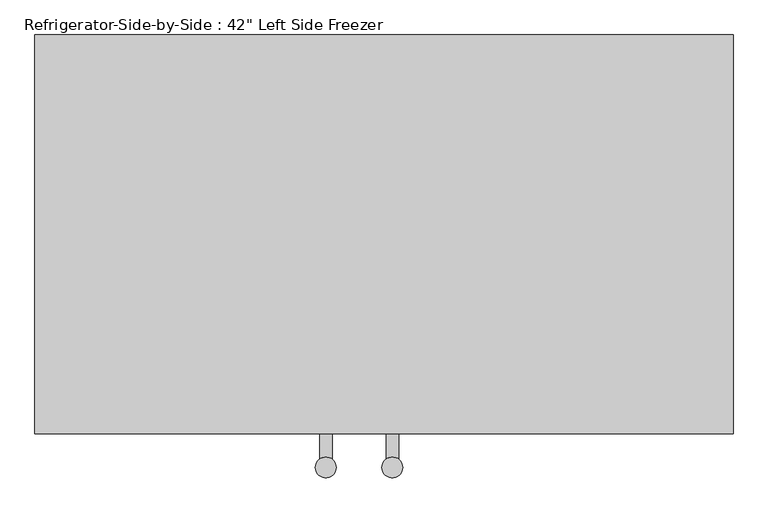
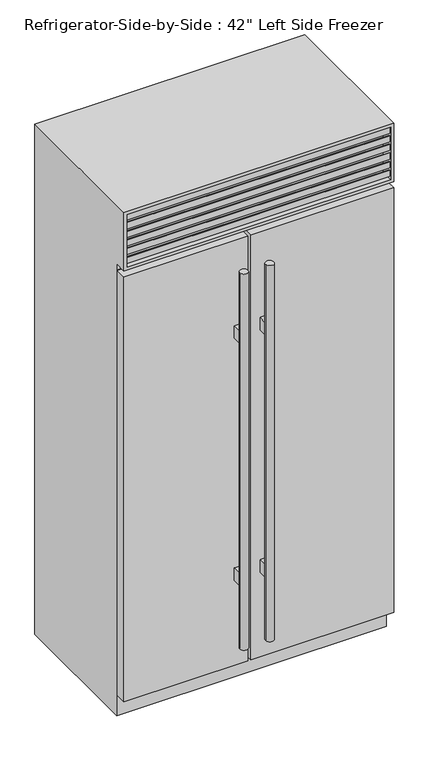
"""IFC4 building model written with IfcOpenShell, lengths in millimetres: proxy geometry."""

from ifc_helpers import new_model, si_unit, frame, origin, place, context, project, spatial, polyline, circle_curve, ellipse_curve, outline, extrude, faceted_brep, source, transform, mapped, element, save
from ifc_brep_helpers import plane_surface, cylinder_surface, advanced_brep


def proxy_0447ab4b(model_context):
    return source(origin(), model_context, "Body", "SolidModel", [
        extrude(outline(polyline([(-533.4, -666.75), (-44.45, -666.75), (-44.45, -711.2), (-533.4, -711.2), (-533.4, -666.75)])), frame((0.0, 0.0, 88.9), z_axis=(0.0, 0.0, 1.0), x_axis=(1.0, 0.0, 0.0)), (0.0, 0.0, 1.0), 1774.825),
        extrude(outline(polyline([(-31.75, -666.75), (533.4, -666.75), (533.4, -711.2), (-31.75, -711.2), (-31.75, -666.75)])), frame((0.0, 0.0, 88.9), z_axis=(0.0, 0.0, 1.0), x_axis=(1.0, 0.0, 0.0)), (0.0, 0.0, 1.0), 1774.825),
        faceted_brep([(533.4, -711.2, 2133.6), (-533.4, -711.2, 2133.6), (-533.4, -711.2, 1889.125), (533.4, -711.2, 1889.125), (520.7, -711.2, 2120.9), (520.7, -711.2, 1901.825), (-520.7, -711.2, 1901.825), (-520.7, -711.2, 2120.9), (533.4, -101.6, 2133.6), (-533.4, -101.6, 2133.6), (-533.4, -101.6, 0.0), (-533.4, -660.4, 0.0), (-533.4, -660.4, 1889.125), (533.4, -660.4, 1889.125), (533.4, -660.4, 0.0), (533.4, -101.6, 0.0), (-520.7, -660.4, 2120.9), (520.7, -660.4, 2120.9), (-520.7, -660.4, 1901.825), (520.7, -660.4, 1901.825)], [[[0, 1, 2, 3], [4, 5, 6, 7]], [[1, 0, 8, 9]], [[2, 1, 9, 10, 11, 12]], [[3, 2, 12, 13]], [[8, 0, 3, 13, 14, 15]], [[4, 7, 16, 17]], [[7, 6, 18, 16]], [[6, 5, 19, 18]], [[5, 4, 17, 19]], [[15, 14, 11, 10]], [[9, 8, 15, 10]], [[17, 16, 18, 19]], [[11, 14, 13, 12]]]),
        extrude(outline(polyline([(-660.4, 1901.825), (-708.025, 1914.5860803), (-708.025, 1939.9860803), (-704.85, 1939.9860803), (-704.85, 1917.1368938), (-660.4, 1905.2265522), (-660.4, 1901.825)])), frame((-520.7, 0.0, 0.0), z_axis=(1.0, 0.0, 0.0), x_axis=(0.0, 1.0, 0.0)), (0.0, 0.0, 1.0), 1041.4),
        extrude(outline(polyline([(-660.4, 1938.0077839), (-708.025, 1950.7688642), (-708.025, 1976.1688642), (-704.85, 1976.1688642), (-704.85, 1953.3196777), (-660.4, 1941.4093361), (-660.4, 1938.0077839)])), frame((-520.7, 0.0, 0.0), z_axis=(1.0, 0.0, 0.0), x_axis=(0.0, 1.0, 0.0)), (0.0, 0.0, 1.0), 1041.4),
        extrude(outline(polyline([(-660.4, 1974.1905679), (-708.025, 1986.9516482), (-708.025, 2012.3516482), (-704.85, 2012.3516482), (-704.85, 1989.5024616), (-660.4, 1977.59212), (-660.4, 1974.1905679)])), frame((-520.7, 0.0, 0.0), z_axis=(1.0, 0.0, 0.0), x_axis=(0.0, 1.0, 0.0)), (0.0, 0.0, 1.0), 1041.4),
        extrude(outline(polyline([(-660.4, 2010.3733518), (-708.025, 2023.1344321), (-708.025, 2048.5344321), (-704.85, 2048.5344321), (-704.85, 2025.6852456), (-660.4, 2013.774904), (-660.4, 2010.3733518)])), frame((-520.7, 0.0, 0.0), z_axis=(1.0, 0.0, 0.0), x_axis=(0.0, 1.0, 0.0)), (0.0, 0.0, 1.0), 1041.4),
        extrude(outline(polyline([(-660.4, 2046.5561358), (-708.025, 2059.3172161), (-708.025, 2084.7172161), (-704.85, 2084.7172161), (-704.85, 2061.8680295), (-660.4, 2049.9576879), (-660.4, 2046.5561358)])), frame((-520.7, 0.0, 0.0), z_axis=(1.0, 0.0, 0.0), x_axis=(0.0, 1.0, 0.0)), (0.0, 0.0, 1.0), 1041.4),
        extrude(outline(polyline([(-660.4, 2082.7389197), (-708.025, 2095.5), (-708.025, 2120.9), (-704.85, 2120.9), (-704.85, 2098.0508135), (-660.4, 2086.1404719), (-660.4, 2082.7389197)])), frame((-520.7, 0.0, 0.0), z_axis=(1.0, 0.0, 0.0), x_axis=(0.0, 1.0, 0.0)), (0.0, 0.0, 1.0), 1041.4),
        advanced_brep(
        [(-25.4, -660.4, 1857.375), (-25.4, -666.75, 1857.375), (-25.4, -666.75, 95.25), (-25.4, -660.4, 95.25), (527.05, -666.75, 95.25), (527.05, -660.4, 95.25), (527.05, -666.75, 1857.375), (527.05, -660.4, 1857.375), (-28.575, -660.4, 1860.55), (530.225, -660.4, 1860.55), (530.225, -660.4, 92.075), (-28.575, -660.4, 92.075), (-28.575, -666.75, 92.075), (530.225, -666.75, 92.075), (530.225, -666.75, 1860.55), (-28.575, -666.75, 1860.55)],
        [
            (0, 1),
            (1, 2),
            (2, 3),
            (3, 0),
            (2, 4),
            (4, 5),
            (5, 3),
            (4, 6),
            (6, 7),
            (7, 5),
            (8, 9),
            (9, 10),
            (10, 11),
            (11, 8),
            (7, 0),
            (12, 13),
            (13, 14),
            (14, 15),
            (15, 12),
            (1, 6),
            (15, 8, ellipse_curve(frame((-28.575, -663.575, 1860.55), z_axis=(-0.7071067811865415, 0.0, -0.7071067811865537), x_axis=(-0.7071067811865536, 0.0, 0.7071067811865414)), 4.4901281, 3.175)),
            (11, 12, ellipse_curve(frame((-28.575, -663.575, 92.075), z_axis=(-0.7071067811865598, 0.0, 0.7071067811865352), x_axis=(0.7071067811865352, 0.0, 0.7071067811865598)), 4.4901281, 3.175)),
            (10, 13, ellipse_curve(frame((530.225, -663.575, 92.075), z_axis=(-0.7071067811865352, 0.0, -0.7071067811865598), x_axis=(-0.7071067811865598, 0.0, 0.7071067811865352)), 4.4901281, 3.175)),
            (9, 14, ellipse_curve(frame((530.225, -663.575, 1860.55), z_axis=(0.7071067811865536, 0.0, -0.7071067811865412), x_axis=(-0.7071067811865411, 0.0, -0.7071067811865539)), 4.4901281, 3.175)),
        ],
        [
            plane_surface(frame((-25.4, -666.75, 1857.375), z_axis=(1.0, 0.0, 0.0), x_axis=(0.0, 0.0, -1.0))),
            plane_surface(frame((-25.4, -666.75, 95.25), z_axis=(0.0, 0.0, 1.0), x_axis=(1.0, 0.0, 0.0))),
            plane_surface(frame((527.05, -666.75, 95.25), z_axis=(-1.0, 0.0, 0.0), x_axis=(0.0, 0.0, 1.0))),
            plane_surface(frame((527.05, -660.4, 1857.375), z_axis=(0.0, 1.0, 0.0), x_axis=(-1.0, 0.0, 0.0))),
            plane_surface(frame((530.225, -666.75, 1860.55), z_axis=(0.0, -1.0, 0.0), x_axis=(-1.0, 0.0, 0.0))),
            plane_surface(frame((527.05, -666.75, 1857.375), z_axis=(0.0, 0.0, -1.0), x_axis=(-1.0, 0.0, 0.0))),
            cylinder_surface(frame((-28.575, -663.575, 1863.725), z_axis=(0.0, 0.0, 1.0), x_axis=(0.0, -1.0, 0.0)), 3.175),
            cylinder_surface(frame((-31.75, -663.575, 92.075), z_axis=(-1.0, 0.0, 0.0), x_axis=(0.0, -1.0, 0.0)), 3.175),
            cylinder_surface(frame((530.225, -663.575, 88.9), z_axis=(0.0, 0.0, -1.0), x_axis=(0.0, -1.0, 0.0)), 3.175),
            cylinder_surface(frame((533.4, -663.575, 1860.55), z_axis=(1.0, 0.0, 0.0), x_axis=(0.0, -1.0, 0.0)), 3.175),
        ],
        [
            (0, [[1, 2, 3, 4]]),
            (1, [[-3, 5, 6, 7]]),
            (2, [[-6, 8, 9, 10]]),
            (3, [[11, 12, 13, 14], [-7, -10, 15, -4]]),
            (4, [[16, 17, 18, 19], [20, -8, -5, -2]]),
            (5, [[-9, -20, -1, -15]]),
            (6, [[21, -14, 22, -19]]),
            (7, [[-22, -13, 23, -16]]),
            (8, [[-23, -12, 24, -17]]),
            (9, [[-24, -11, -21, -18]]),
        ],
    ),
        advanced_brep(
        [(-527.05, -660.4, 1857.375), (-527.05, -666.75, 1857.375), (-527.05, -666.75, 95.25), (-527.05, -660.4, 95.25), (-50.8, -666.75, 95.25), (-50.8, -660.4, 95.25), (-50.8, -666.75, 1857.375), (-50.8, -660.4, 1857.375), (-530.225, -660.4, 1860.55), (-47.625, -660.4, 1860.55), (-47.625, -660.4, 92.075), (-530.225, -660.4, 92.075), (-530.225, -666.75, 92.075), (-47.625, -666.75, 92.075), (-47.625, -666.75, 1860.55), (-530.225, -666.75, 1860.55)],
        [
            (0, 1),
            (1, 2),
            (2, 3),
            (3, 0),
            (2, 4),
            (4, 5),
            (5, 3),
            (4, 6),
            (6, 7),
            (7, 5),
            (8, 9),
            (9, 10),
            (10, 11),
            (11, 8),
            (7, 0),
            (12, 13),
            (13, 14),
            (14, 15),
            (15, 12),
            (1, 6),
            (15, 8, ellipse_curve(frame((-530.225, -663.575, 1860.55), z_axis=(-0.7071067811865475, 0.0, -0.7071067811865475), x_axis=(-0.7071067811865474, 0.0, 0.7071067811865476)), 4.4901281, 3.175)),
            (11, 12, ellipse_curve(frame((-530.225, -663.575, 92.075), z_axis=(-0.7071067811865475, 0.0, 0.7071067811865475), x_axis=(0.7071067811865474, 0.0, 0.7071067811865476)), 4.4901281, 3.175)),
            (10, 13, ellipse_curve(frame((-47.625, -663.575, 92.075), z_axis=(-0.7071067811865475, 0.0, -0.7071067811865475), x_axis=(-0.7071067811865476, 0.0, 0.7071067811865474)), 4.4901281, 3.175)),
            (9, 14, ellipse_curve(frame((-47.625, -663.575, 1860.55), z_axis=(0.7071067811865475, 0.0, -0.7071067811865475), x_axis=(-0.7071067811865474, 0.0, -0.7071067811865476)), 4.4901281, 3.175)),
        ],
        [
            plane_surface(frame((-527.05, -666.75, 1857.375), z_axis=(1.0, 0.0, 0.0), x_axis=(0.0, 0.0, -1.0))),
            plane_surface(frame((-527.05, -666.75, 95.25), z_axis=(0.0, 0.0, 1.0), x_axis=(1.0, 0.0, 0.0))),
            plane_surface(frame((-50.8, -666.75, 95.25), z_axis=(-1.0, 0.0, 0.0), x_axis=(0.0, 0.0, 1.0))),
            plane_surface(frame((-50.8, -660.4, 1857.375), z_axis=(0.0, 1.0, 0.0), x_axis=(-1.0, 0.0, 0.0))),
            plane_surface(frame((-47.625, -666.75, 1860.55), z_axis=(0.0, -1.0, 0.0), x_axis=(-1.0, 0.0, 0.0))),
            plane_surface(frame((-50.8, -666.75, 1857.375), z_axis=(0.0, 0.0, -1.0), x_axis=(-1.0, 0.0, 0.0))),
            cylinder_surface(frame((-530.225, -663.575, 1863.725), z_axis=(0.0, 0.0, 1.0), x_axis=(0.0, -1.0, 0.0)), 3.175),
            cylinder_surface(frame((-533.4, -663.575, 92.075), z_axis=(-1.0, 0.0, 0.0), x_axis=(0.0, -1.0, 0.0)), 3.175),
            cylinder_surface(frame((-47.625, -663.575, 88.9), z_axis=(0.0, 0.0, -1.0), x_axis=(0.0, -1.0, 0.0)), 3.175),
            cylinder_surface(frame((-44.45, -663.575, 1860.55), z_axis=(1.0, 0.0, 0.0), x_axis=(0.0, -1.0, 0.0)), 3.175),
        ],
        [
            (0, [[1, 2, 3, 4]]),
            (1, [[-3, 5, 6, 7]]),
            (2, [[-6, 8, 9, 10]]),
            (3, [[11, 12, 13, 14], [-7, -10, 15, -4]]),
            (4, [[16, 17, 18, 19], [20, -8, -5, -2]]),
            (5, [[-9, -20, -1, -15]]),
            (6, [[21, -14, 22, -19]]),
            (7, [[-22, -13, 23, -16]]),
            (8, [[-23, -12, 24, -17]]),
            (9, [[-24, -11, -21, -18]]),
        ],
    ),
        advanced_brep(
        [(-3.175, -762.3741958, 1762.125), (28.575, -762.3741958, 1762.125), (-3.175, -762.3741958, 190.5), (28.575, -762.3741958, 190.5), (22.225, -749.6741958, 1457.325), (22.225, -749.6741958, 1508.125), (3.175, -749.6741958, 1508.125), (3.175, -749.6741958, 1457.325), (22.225, -749.6741958, 444.5), (22.225, -749.6741958, 495.3), (3.175, -749.6741958, 495.3), (3.175, -749.6741958, 444.5), (22.225, -711.2, 1508.125), (22.225, -711.2, 1457.325), (3.175, -711.2, 1457.325), (3.175, -711.2, 1508.125), (22.225, -711.2, 495.3), (22.225, -711.2, 444.5), (3.175, -711.2, 444.5), (3.175, -711.2, 495.3)],
        [
            (0, 1, circle_curve(frame((12.7, -762.3741958, 1762.125), z_axis=(0.0, 0.0, 1.0), x_axis=(1.0, 0.0, 0.0)), 15.875)),
            (1, 0, circle_curve(frame((12.7, -762.3741958, 1762.125), z_axis=(0.0, 0.0, 1.0), x_axis=(1.0, 0.0, 0.0)), 15.875)),
            (2, 3, circle_curve(frame((12.7, -762.3741958, 190.5), z_axis=(0.0, 0.0, -1.0), x_axis=(1.0, 0.0, 0.0)), 15.875)),
            (3, 2, circle_curve(frame((12.7, -762.3741958, 190.5), z_axis=(0.0, 0.0, -1.0), x_axis=(1.0, 0.0, 0.0)), 15.875)),
            (0, 2),
            (3, 1),
            (4, 5),
            (5, 6, circle_curve(frame((12.7, -762.3741958, 1508.125), z_axis=(0.0, 0.0, 1.0), x_axis=(1.0, 0.0, 0.0)), 15.875)),
            (6, 7),
            (7, 4, circle_curve(frame((12.7, -762.3741958, 1457.325), z_axis=(0.0, 0.0, -1.0), x_axis=(1.0, 0.0, 0.0)), 15.875)),
            (8, 9),
            (9, 10, circle_curve(frame((12.7, -762.3741958, 495.3), z_axis=(0.0, 0.0, 1.0), x_axis=(1.0, 0.0, 0.0)), 15.875)),
            (10, 11),
            (11, 8, circle_curve(frame((12.7, -762.3741958, 444.5), z_axis=(0.0, 0.0, -1.0), x_axis=(1.0, 0.0, 0.0)), 15.875)),
            (12, 13),
            (13, 14),
            (14, 15),
            (15, 12),
            (16, 17),
            (17, 18),
            (18, 19),
            (19, 16),
            (12, 5),
            (4, 13),
            (7, 14),
            (6, 15),
            (16, 9),
            (8, 17),
            (11, 18),
            (10, 19),
        ],
        [
            plane_surface(frame((28.575, -762.3741958, 1762.125), z_axis=(0.0, 0.0, 1.0), x_axis=(0.0, 1.0, 0.0))),
            plane_surface(frame((28.575, -762.3741958, 190.5), z_axis=(0.0, 0.0, -1.0), x_axis=(0.0, -1.0, 0.0))),
            cylinder_surface(frame((12.7, -762.3741958, 190.5), z_axis=(0.0, 0.0, 1.0), x_axis=(1.0, 0.0, 0.0)), 15.875),
            plane_surface(frame((22.225, -711.2, 1508.125), z_axis=(0.0, 1.0, 0.0), x_axis=(0.0, 0.0, -1.0))),
            plane_surface(frame((22.225, -711.2, 1508.125), z_axis=(1.0, 0.0, 0.0), x_axis=(0.0, -1.0, 0.0))),
            plane_surface(frame((22.225, -711.2, 1457.325), z_axis=(0.0, 0.0, -1.0), x_axis=(0.0, -1.0, 0.0))),
            plane_surface(frame((3.175, -711.2, 1457.325), z_axis=(-1.0, 0.0, 0.0), x_axis=(0.0, -1.0, 0.0))),
            plane_surface(frame((3.175, -711.2, 1508.125), z_axis=(0.0, 0.0, 1.0), x_axis=(0.0, -1.0, 0.0))),
            plane_surface(frame((22.225, -711.2, 495.3), z_axis=(1.0, 0.0, 0.0), x_axis=(0.0, -1.0, 0.0))),
            plane_surface(frame((22.225, -711.2, 444.5), z_axis=(0.0, 0.0, -1.0), x_axis=(0.0, -1.0, 0.0))),
            plane_surface(frame((3.175, -711.2, 444.5), z_axis=(-1.0, 0.0, 0.0), x_axis=(0.0, -1.0, 0.0))),
            plane_surface(frame((3.175, -711.2, 495.3), z_axis=(0.0, 0.0, 1.0), x_axis=(0.0, -1.0, 0.0))),
        ],
        [
            (0, [[1, 2]]),
            (1, [[3, 4]]),
            (2, [[-1, 5, -4, 6]]),
            (2, [[-2, -6, -3, -5], [7, 8, 9, 10], [11, 12, 13, 14]]),
            (3, [[15, 16, 17, 18]]),
            (3, [[19, 20, 21, 22]]),
            (4, [[-15, 23, -7, 24]]),
            (5, [[-16, -24, -10, 25]]),
            (6, [[-17, -25, -9, 26]]),
            (7, [[-18, -26, -8, -23]]),
            (8, [[-19, 27, -11, 28]]),
            (9, [[-20, -28, -14, 29]]),
            (10, [[-21, -29, -13, 30]]),
            (11, [[-22, -30, -12, -27]]),
        ],
    ),
        advanced_brep(
        [(-79.375, -711.2, 1508.125), (-79.375, -711.2, 1457.325), (-98.425, -711.2, 1457.325), (-98.425, -711.2, 1508.125), (-79.375, -711.2, 495.3), (-79.375, -711.2, 444.5), (-98.425, -711.2, 444.5), (-98.425, -711.2, 495.3), (-79.375, -749.6741958, 1508.125), (-79.375, -749.6741958, 1457.325), (-98.425, -749.6741958, 1457.325), (-98.425, -749.6741958, 1508.125), (-79.375, -749.6741958, 495.3), (-79.375, -749.6741958, 444.5), (-98.425, -749.6741958, 444.5), (-98.425, -749.6741958, 495.3), (-104.775, -762.3741958, 1762.125), (-73.025, -762.3741958, 1762.125), (-104.775, -762.3741958, 190.5), (-73.025, -762.3741958, 190.5)],
        [
            (0, 1),
            (1, 2),
            (2, 3),
            (3, 0),
            (4, 5),
            (5, 6),
            (6, 7),
            (7, 4),
            (0, 8),
            (8, 9),
            (9, 1),
            (9, 10, circle_curve(frame((-88.9, -762.3741958, 1457.325), z_axis=(0.0, 0.0, 1.0), x_axis=(1.0, 0.0, 0.0)), 15.875)),
            (10, 2),
            (10, 11),
            (11, 3),
            (11, 8, circle_curve(frame((-88.9, -762.3741958, 1508.125), z_axis=(0.0, 0.0, -1.0), x_axis=(1.0, 0.0, 0.0)), 15.875)),
            (4, 12),
            (12, 13),
            (13, 5),
            (13, 14, circle_curve(frame((-88.9, -762.3741958, 444.5), z_axis=(0.0, 0.0, 1.0), x_axis=(1.0, 0.0, 0.0)), 15.875)),
            (14, 6),
            (14, 15),
            (15, 7),
            (15, 12, circle_curve(frame((-88.9, -762.3741958, 495.3), z_axis=(0.0, 0.0, -1.0), x_axis=(1.0, 0.0, 0.0)), 15.875)),
            (16, 17, circle_curve(frame((-88.9, -762.3741958, 1762.125), z_axis=(0.0, 0.0, 1.0), x_axis=(1.0, 0.0, 0.0)), 15.875)),
            (17, 16, circle_curve(frame((-88.9, -762.3741958, 1762.125), z_axis=(0.0, 0.0, 1.0), x_axis=(1.0, 0.0, 0.0)), 15.875)),
            (18, 19, circle_curve(frame((-88.9, -762.3741958, 190.5), z_axis=(0.0, 0.0, -1.0), x_axis=(1.0, 0.0, 0.0)), 15.875)),
            (19, 18, circle_curve(frame((-88.9, -762.3741958, 190.5), z_axis=(0.0, 0.0, -1.0), x_axis=(1.0, 0.0, 0.0)), 15.875)),
            (16, 18),
            (19, 17),
        ],
        [
            plane_surface(frame((-79.375, -711.2, 1508.125), z_axis=(0.0, 1.0, 0.0), x_axis=(0.0, 0.0, -1.0))),
            plane_surface(frame((-79.375, -711.2, 1508.125), z_axis=(1.0, 0.0, 0.0), x_axis=(0.0, -1.0, 0.0))),
            plane_surface(frame((-79.375, -711.2, 1457.325), z_axis=(0.0, 0.0, -1.0), x_axis=(0.0, -1.0, 0.0))),
            plane_surface(frame((-98.425, -711.2, 1457.325), z_axis=(-1.0, 0.0, 0.0), x_axis=(0.0, -1.0, 0.0))),
            plane_surface(frame((-98.425, -711.2, 1508.125), z_axis=(0.0, 0.0, 1.0), x_axis=(0.0, -1.0, 0.0))),
            plane_surface(frame((-79.375, -711.2, 495.3), z_axis=(1.0, 0.0, 0.0), x_axis=(0.0, -1.0, 0.0))),
            plane_surface(frame((-79.375, -711.2, 444.5), z_axis=(0.0, 0.0, -1.0), x_axis=(0.0, -1.0, 0.0))),
            plane_surface(frame((-98.425, -711.2, 444.5), z_axis=(-1.0, 0.0, 0.0), x_axis=(0.0, -1.0, 0.0))),
            plane_surface(frame((-98.425, -711.2, 495.3), z_axis=(0.0, 0.0, 1.0), x_axis=(0.0, -1.0, 0.0))),
            plane_surface(frame((-73.025, -762.3741958, 1762.125), z_axis=(0.0, 0.0, 1.0), x_axis=(0.0, 1.0, 0.0))),
            plane_surface(frame((-73.025, -762.3741958, 190.5), z_axis=(0.0, 0.0, -1.0), x_axis=(0.0, -1.0, 0.0))),
            cylinder_surface(frame((-88.9, -762.3741958, 190.5), z_axis=(0.0, 0.0, 1.0), x_axis=(1.0, 0.0, 0.0)), 15.875),
        ],
        [
            (0, [[1, 2, 3, 4]]),
            (0, [[5, 6, 7, 8]]),
            (1, [[-1, 9, 10, 11]]),
            (2, [[-2, -11, 12, 13]]),
            (3, [[-3, -13, 14, 15]]),
            (4, [[-4, -15, 16, -9]]),
            (5, [[-5, 17, 18, 19]]),
            (6, [[-6, -19, 20, 21]]),
            (7, [[-7, -21, 22, 23]]),
            (8, [[-8, -23, 24, -17]]),
            (9, [[25, 26]]),
            (10, [[27, 28]]),
            (11, [[-25, 29, -28, 30]]),
            (11, [[-26, -30, -27, -29], [-10, -16, -14, -12], [-18, -24, -22, -20]]),
        ],
    ),
    ])


if __name__ == "__main__":
    model = new_model("IFC4")
    model_context = context("Model", 3, world=origin())
    ifc_project = project(units=[si_unit("LENGTHUNIT", "METRE", prefix="MILLI")], contexts=[model_context])
    site = spatial("IfcSite", under=ifc_project)
    building = spatial("IfcBuilding", under=site)
    placement = place(None, origin())
    proxy_shape = proxy_0447ab4b(model_context)
    element("IfcBuildingElementProxy", 1, Name="Refrigerator-Side-by-Side : 42\" Left Side Freezer", ObjectType="Refrigerator-Side-by-Side : 42\" Left Side Freezer", at=placement, inside=building, context=model_context, shape_type="MappedRepresentation", body=[
        mapped(proxy_shape, transform((0.0, 0.0, 0.0), x_axis=(1.0, 0.0, 0.0), y_axis=(0.0, 1.0, 0.0), z_axis=(0.0, 0.0, 1.0))),
    ])
    save(model, "model.ifc")

# Revit data of these elements
# Type "Refrigerator-Side-by-Side : 42\" Left Side Freezer"
#   Label = "Refrigerator"
#   Description = "Side-by-Side Refrigerator"
#   Assembly Code = "E1090320"
#   Right Door Width = 1' - 10 1/4"
#   Left Door Width = 1' - 7 1/4"
#   Width = 3' - 6"
#   Wall Offset = 0' - 4"
#   Voltage = 120 V
#   Power Consumption = 1000 VA
#   Height = 7' - 0"
#   Door Location = 1' - 7 1/2"
#   Depth = 2' - 0"
#   Amperage = 8.33333 A
#   Show Label = yes
#   Gasket = Appliance - Gasket
#   Appliance Finish = Appliance - Stainless Steel
#   Default Elevation = 0
# Element 1 (IfcBuildingElementProxy, "Refrigerator-Side-by-Side : 42\" Left Side Freezer")
#   Materials on its faces: "Appliance - Stainless Steel", "Appliance - Gasket"
# Materials
#   "Appliance - Gasket": class "Miscellaneous", colour RGB 234 234 234, transparency 0, Cost = 0
#   "Appliance - Stainless Steel": class "Metal", colour RGB 189 187 185, transparency 0, Description = "Stainless Steel 18/8", Cost = 0
